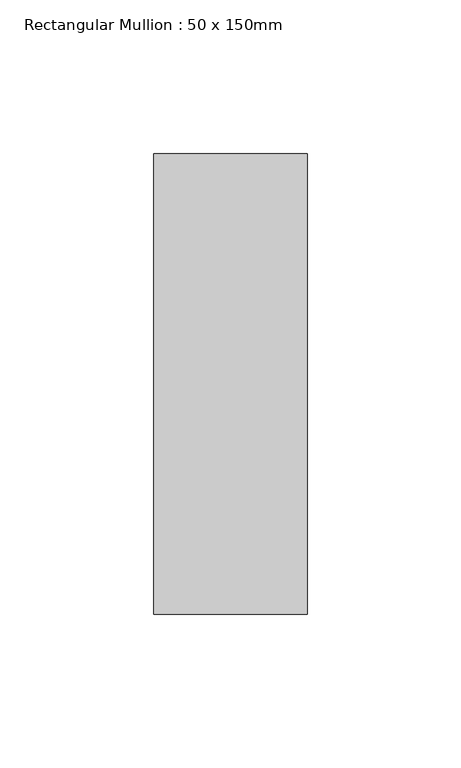
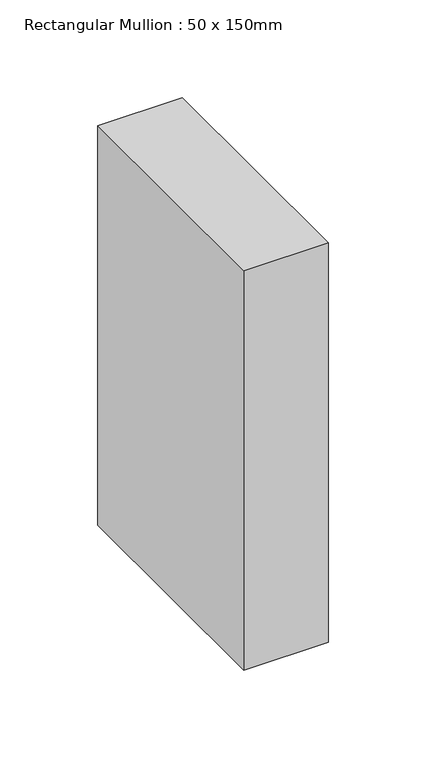
"""IFC4 building model written with IfcOpenShell, lengths in millimetres: member geometry, Rectangular Mullion : 50 x 150mm."""

from ifc_helpers import new_model, si_unit, frame, origin, place, context, project, spatial, polyline, outline, extrude, source, transform, mapped, element, save


def rectangular_mullion_50_x_150mm_43431b2b(model_context):
    return source(origin(), model_context, "Body", "SweptSolid", [
        extrude(outline(polyline([(0.0, 75.0), (0.0, -75.0), (-50.0, -75.0), (-50.0, 75.0), (0.0, 75.0)])), frame((0.0, 0.0, -250.0000002), z_axis=(0.0, 0.0, 1.0), x_axis=(1.0, 0.0, 0.0)), (0.0, 0.0, 1.0), 250.0000002),
    ])


if __name__ == "__main__":
    model = new_model("IFC4")
    model_context = context("Model", 3, world=origin())
    ifc_project = project(units=[si_unit("LENGTHUNIT", "METRE", prefix="MILLI")], contexts=[model_context])
    site = spatial("IfcSite", under=ifc_project)
    building = spatial("IfcBuilding", under=site)
    placement = place(None, origin())
    rectangular_mullion_50_x_150mm_shape = rectangular_mullion_50_x_150mm_43431b2b(model_context)
    element("IfcMember", 1, ObjectType="Rectangular Mullion : 50 x 150mm", at=placement, inside=building, context=model_context, shape_type="MappedRepresentation", body=[
        mapped(rectangular_mullion_50_x_150mm_shape, transform((0.0, 0.0, 0.0), x_axis=(1.0, 0.0, 0.0), y_axis=(0.0, 1.0, 0.0), z_axis=(0.0, 0.0, 1.0))),
    ])
    save(model, "model.ifc")

# Revit data of these elements
# Type "Rectangular Mullion : 50 x 150mm"
#   built-in parameter 1007304 = 0.492126 (stored number, unit not read)
#   built-in parameter 1007301 = 0.082021 (stored number, unit not read)
#   built-in parameter 1007300 = 0.082021 (stored number, unit not read)
# Element 1 (IfcMember, "Rectangular Mullion : 50 x 150mm")
#   Materials on its faces: "Aluminium"
# Materials
#   "Aluminium": class "Metal", colour RGB 247 247 247, transparency 0, Description = "Aluminium 6061", Cost = 0
